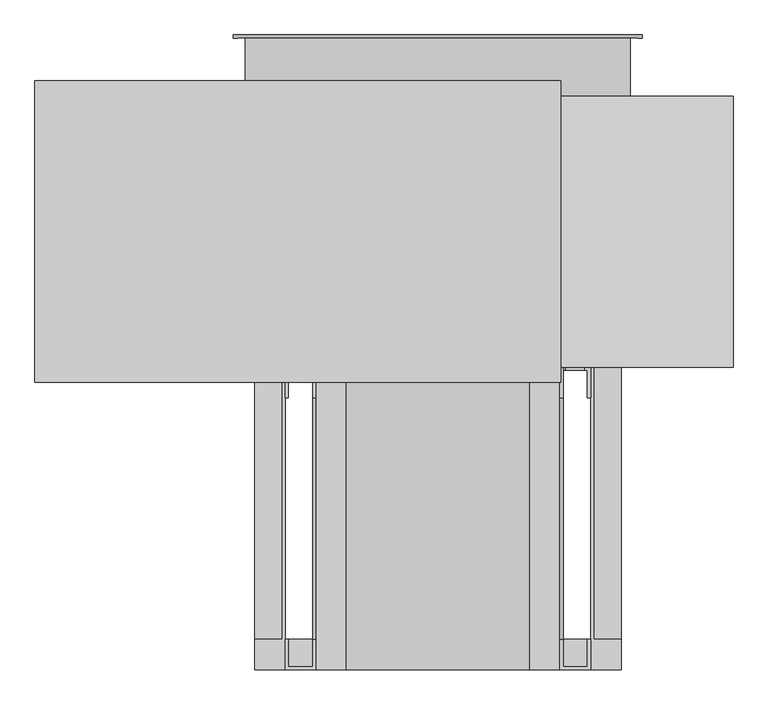
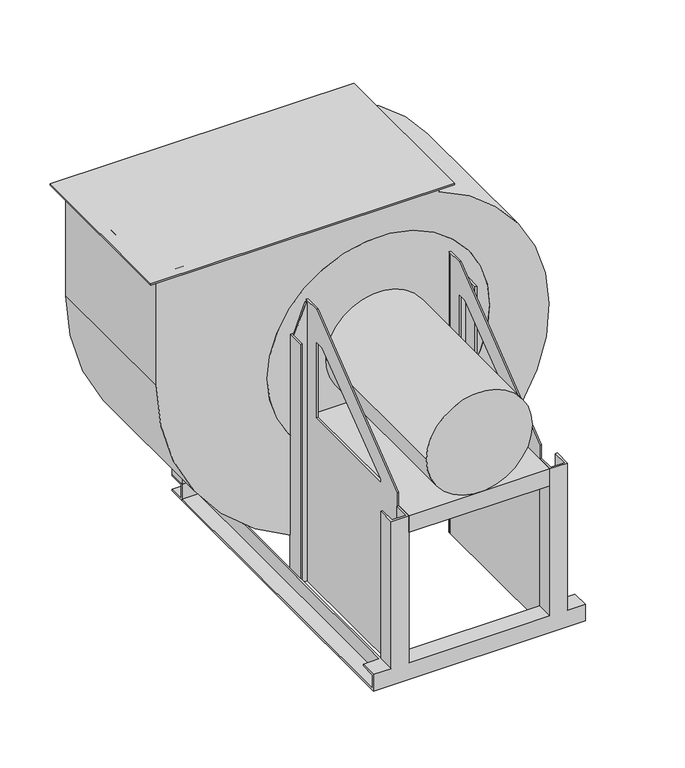
"""IFC4 building model written with IfcOpenShell, lengths in millimetres: proxy geometry, ВЕЗА_Вентилятор ВРАН : ВРАН9-063-ЛО."""

from ifc_helpers import new_model, si_unit, point, frame, frame_2d, origin, place, context, project, spatial, polyline, circle_curve, trimmed, segment, composite_curve, outline, extrude, faceted_brep, source, transform, mapped, element, save


def mechanical_equipment_c4a9a316(model_context):
    return source(origin(), model_context, "Body", "SolidModel", [
        extrude(outline(polyline([(201.5, -247.0), (-659.5, -247.0), (-659.5, 247.0), (201.5, 247.0), (201.5, -247.0)])), frame((0.0, 0.0, 1055.0), z_axis=(0.0, 0.0, 1.0), x_axis=(1.0, 0.0, 0.0)), (0.0, 0.0, 1.0), 5.0),
        extrude(outline(composite_curve([segment(trimmed(circle_curve(frame_2d((730.0, 5.524027)), 635.024027), [point((730.0, -629.5))], [point((95.0, 0.0))], False, "CARTESIAN"), True, "CONTINUOUS"), segment(trimmed(circle_curve(frame_2d((578.1699763, 0.3189338)), 483.1700816), [point((95.0, 0.0))], [point((1030.0, 171.5))], False, "CARTESIAN"), True, "CONTINUOUS"), segment(polyline([(1030.0, 171.5), (1060.0, 171.5), (1060.0, -629.5), (730.0, -629.5)]), True, "CONTINUOUS")], self_intersect=False), holes=[composite_curve([segment(trimmed(circle_curve(frame_2d((640.0, 0.0)), 315.0), [point((640.0, -315.0))], [point((640.0, 315.0))], True, "CARTESIAN"), True, "CONTINUOUS"), segment(trimmed(circle_curve(frame_2d((640.0, 0.0)), 315.0), [point((640.0, 315.0))], [point((640.0, -315.0))], True, "CARTESIAN"), True, "CONTINUOUS")], self_intersect=False)]), frame((0.0, -222.0, 0.0), z_axis=(0.0, 1.0, 0.0), x_axis=(0.0, 0.0, 1.0)), (0.0, 0.0, 1.0), 444.0),
        faceted_brep([(-300.0, -712.0, 5.0), (-300.0, 222.0, 5.0), (-300.0, 222.0, 0.0), (-300.0, -717.0, 0.0), (-300.0, -717.0, 50.0), (-300.0, -667.0, 50.0), (-300.0, -667.0, 45.0), (-300.0, -712.0, 45.0), (300.0, -717.0, 50.0), (300.0, -717.0, 0.0), (300.0, 222.0, 0.0), (300.0, 222.0, 5.0), (300.0, -712.0, 5.0), (300.0, -712.0, 45.0), (300.0, -667.0, 45.0), (300.0, -667.0, 50.0), (-250.0, 222.0, 0.0), (-250.0, -667.0, 0.0), (250.0, -667.0, 0.0), (250.0, 222.0, 0.0), (-255.0, -667.0, 50.0), (-255.0, -667.0, 45.0), (255.0, -667.0, 45.0), (255.0, -667.0, 50.0), (-200.0, -667.0, 490.0), (-200.0, -667.0, 50.0), (200.0, -667.0, 50.0), (200.0, -667.0, 490.0), (205.0, -667.0, 490.0), (205.0, -667.0, 50.0), (245.0, -667.0, 50.0), (245.0, -667.0, 490.0), (250.0, -667.0, 490.0), (250.0, -667.0, 50.0), (-250.0, -667.0, 50.0), (-250.0, -667.0, 490.0), (-245.0, -667.0, 490.0), (-245.0, -667.0, 50.0), (-205.0, -667.0, 50.0), (-205.0, -667.0, 490.0), (205.0, -667.0, 5.0), (245.0, -667.0, 5.0), (245.0, -667.0, 45.0), (205.0, -667.0, 45.0), (-245.0, -667.0, 5.0), (-205.0, -667.0, 5.0), (-205.0, -667.0, 45.0), (-245.0, -667.0, 45.0), (-200.0, -667.0, 5.0), (200.0, -667.0, 5.0), (200.0, -667.0, 45.0), (-200.0, -667.0, 45.0), (-255.0, -712.0, 5.0), (-255.0, 222.0, 5.0), (255.0, 222.0, 5.0), (255.0, -712.0, 5.0), (205.0, -712.0, 5.0), (245.0, -712.0, 5.0), (-245.0, -712.0, 5.0), (-205.0, -712.0, 5.0), (-200.0, -712.0, 5.0), (200.0, -712.0, 5.0), (255.0, -712.0, 45.0), (-255.0, -712.0, 45.0), (205.0, -712.0, 45.0), (245.0, -712.0, 45.0), (-245.0, -712.0, 45.0), (-205.0, -712.0, 45.0), (-200.0, -712.0, 45.0), (200.0, -712.0, 45.0), (255.0, 222.0, 50.0), (250.0, 222.0, 50.0), (250.0, -717.0, 50.0), (-250.0, -717.0, 50.0), (-250.0, 222.0, 50.0), (-255.0, 222.0, 50.0), (205.0, -712.0, 50.0), (245.0, -712.0, 50.0), (-245.0, -712.0, 50.0), (-205.0, -712.0, 50.0), (-200.0, -717.0, 50.0), (200.0, -717.0, 50.0), (250.0, -717.0, 490.0), (200.0, -717.0, 490.0), (-200.0, -717.0, 490.0), (-250.0, -717.0, 490.0), (245.0, -712.0, 490.0), (205.0, -712.0, 490.0), (-205.0, -712.0, 490.0), (-245.0, -712.0, 490.0)], [[[0, 1, 2, 3, 4, 5, 6, 7]], [[8, 9, 10, 11, 12, 13, 14, 15]], [[10, 9, 3, 2, 16, 17, 18, 19]], [[5, 20, 21, 6]], [[14, 22, 23, 15]], [[24, 25, 26, 27, 28, 29, 30, 31, 32, 33, 18, 17, 34, 35, 36, 37, 38, 39], [40, 41, 42, 43], [44, 45, 46, 47], [48, 49, 50, 51]], [[1, 0, 52, 53]], [[54, 55, 12, 11]], [[40, 56, 57, 41]], [[44, 58, 59, 45]], [[48, 60, 61, 49]], [[12, 55, 62, 13]], [[7, 63, 52, 0]], [[56, 64, 65, 57]], [[58, 66, 67, 59]], [[60, 68, 69, 61]], [[6, 21, 63, 7]], [[13, 62, 22, 14]], [[64, 43, 42, 65]], [[66, 47, 46, 67]], [[68, 51, 50, 69]], [[15, 23, 70, 71, 33, 72, 8]], [[4, 73, 34, 74, 75, 20, 5]], [[29, 76, 77, 30]], [[37, 78, 79, 38]], [[25, 80, 81, 26]], [[8, 72, 82, 83, 81, 80, 84, 85, 73, 4, 3, 9]], [[70, 54, 11, 10, 19, 71]], [[70, 23, 22, 62, 55, 54]], [[19, 18, 33, 71]], [[75, 74, 16, 2, 1, 53]], [[53, 52, 63, 21, 20, 75]], [[74, 34, 17, 16]], [[83, 82, 32, 31, 86, 87, 28, 27]], [[84, 24, 39, 88, 89, 36, 35, 85]], [[86, 77, 76, 87]], [[31, 30, 77, 86]], [[41, 57, 65, 42]], [[82, 72, 33, 32]], [[27, 26, 81, 83]], [[49, 61, 69, 50]], [[43, 64, 56, 40]], [[87, 76, 29, 28]], [[35, 34, 73, 85]], [[47, 66, 58, 44]], [[89, 78, 37, 36]], [[88, 79, 78, 89]], [[39, 38, 79, 88]], [[45, 59, 67, 46]], [[51, 68, 60, 48]], [[84, 80, 25, 24]]]),
        extrude(outline(polyline([(-667.0, 0.0), (-667.0, 530.0420316), (-272.0420316, 840.0), (-222.0, 840.0), (-222.0, 0.0), (-667.0, 0.0)]), holes=[polyline([(-272.0, 515.0), (-272.0, 740.0), (-296.9504813, 740.0), (-587.0, 521.5949723), (-587.0, 515.0), (-272.0, 515.0)])]), frame((-205.0, 0.0, 0.0), z_axis=(1.0, 0.0, 0.0), x_axis=(0.0, 1.0, 0.0)), (0.0, 0.0, 1.0), 5.0),
        faceted_brep([(250.0, 222.0, 50.0), (250.0, 227.0, 50.0), (295.0, 227.0, 50.0), (295.0, 272.0, 50.0), (300.0, 272.0, 50.0), (300.0, 222.0, 50.0), (300.0, 222.0, 485.0), (289.966699, 222.0, 485.0), (258.2904546, 222.0, 390.0), (250.0, 222.0, 390.0), (300.0, 272.0, 485.0), (295.0, 272.0, 485.0), (295.0, 227.0, 485.0), (250.0, 227.0, 390.0), (258.2904546, 227.0, 390.0), (289.966699, 227.0, 485.0)], [[[0, 1, 2, 3, 4, 5]], [[5, 6, 7, 8, 9, 0]], [[4, 10, 6, 5]], [[3, 11, 10, 4]], [[2, 12, 11, 3]], [[1, 13, 14, 15, 12, 2]], [[0, 9, 13, 1]], [[14, 13, 9, 8]], [[8, 7, 15, 14]], [[7, 6, 10, 11, 12, 15]]]),
        faceted_brep([(-250.0, 222.0, 50.0), (-300.0, 222.0, 50.0), (-300.0, 272.0, 50.0), (-295.0, 272.0, 50.0), (-295.0, 227.0, 50.0), (-250.0, 227.0, 50.0), (-250.0, 227.0, 390.0), (-250.0, 222.0, 390.0), (-295.0, 227.0, 485.0), (-289.966699, 227.0, 485.0), (-258.2904546, 227.0, 390.0), (-295.0, 272.0, 485.0), (-300.0, 272.0, 485.0), (-300.0, 222.0, 485.0), (-258.2904546, 222.0, 390.0), (-289.966699, 222.0, 485.0)], [[[0, 1, 2, 3, 4, 5]], [[5, 6, 7, 0]], [[4, 8, 9, 10, 6, 5]], [[3, 11, 8, 4]], [[2, 12, 11, 3]], [[1, 13, 12, 2]], [[0, 7, 14, 15, 13, 1]], [[9, 8, 11, 12, 13, 15]], [[15, 14, 10, 9]], [[14, 7, 6, 10]]]),
        extrude(outline(polyline([(-667.0, 0.0), (-667.0, 530.0420316), (-272.0420316, 840.0), (-222.0, 840.0), (-222.0, 0.0), (-667.0, 0.0)]), holes=[polyline([(-272.0, 515.0), (-272.0, 740.0), (-296.9504813, 740.0), (-587.0, 521.5949723), (-587.0, 515.0), (-272.0, 515.0)])]), frame((200.0, 0.0, 0.0), z_axis=(1.0, 0.0, 0.0), x_axis=(0.0, 1.0, 0.0)), (0.0, 0.0, 1.0), 5.0),
        faceted_brep([(200.0, -222.0, 0.0), (250.0, -222.0, 0.0), (250.0, -272.0, 0.0), (245.0, -272.0, 0.0), (245.0, -227.0, 0.0), (200.0, -227.0, 0.0), (200.0, -222.0, 833.6095143), (208.75409, -222.0, 833.6095143), (240.0, -222.0, 750.0), (250.0, -222.0, 750.0), (250.0, -272.0, 750.0), (245.0, -272.0, 750.0), (245.0, -227.0, 750.0), (240.0, -227.0, 750.0), (208.75409, -227.0, 833.6095143), (200.0, -227.0, 833.6095143)], [[[0, 1, 2, 3, 4, 5]], [[0, 6, 7, 8, 9, 1]], [[1, 9, 10, 2]], [[2, 10, 11, 3]], [[3, 11, 12, 4]], [[4, 12, 13, 14, 15, 5]], [[5, 15, 6, 0]], [[7, 6, 15, 14]], [[14, 13, 8, 7]], [[13, 12, 11, 10, 9, 8]]]),
        faceted_brep([(-200.0, -222.0, 0.0), (-200.0, -227.0, 0.0), (-245.0, -227.0, 0.0), (-245.0, -272.0, 0.0), (-250.0, -272.0, 0.0), (-250.0, -222.0, 0.0), (-200.0, -222.0, 833.6095143), (-200.0, -227.0, 833.6095143), (-208.75409, -227.0, 833.6095143), (-240.0, -227.0, 750.0), (-245.0, -227.0, 750.0), (-245.0, -272.0, 750.0), (-250.0, -272.0, 750.0), (-250.0, -222.0, 750.0), (-240.0, -222.0, 750.0), (-208.75409, -222.0, 833.6095143)], [[[0, 1, 2, 3, 4, 5]], [[0, 6, 7, 1]], [[1, 7, 8, 9, 10, 2]], [[2, 10, 11, 3]], [[3, 11, 12, 4]], [[4, 12, 13, 5]], [[5, 13, 14, 15, 6, 0]], [[14, 13, 12, 11, 10, 9]], [[9, 8, 15, 14]], [[8, 7, 6, 15]]]),
        extrude(outline(polyline([(222.0, 50.0), (272.0, 50.0), (272.0, 45.0), (227.0, 45.0), (227.0, 5.0), (272.0, 5.0), (272.0, 0.0), (222.0, 0.0), (222.0, 50.0)])), frame((-300.0, 0.0, 0.0), z_axis=(1.0, 0.0, 0.0), x_axis=(0.0, 1.0, 0.0)), (0.0, 0.0, 1.0), 600.0),
        extrude(outline(composite_curve([segment(trimmed(circle_curve(frame_2d((640.0, 0.0)), 315.0), [point((640.0, -315.0))], [point((640.0, 315.0))], False, "CARTESIAN"), True, "CONTINUOUS"), segment(trimmed(circle_curve(frame_2d((640.0, 0.0)), 315.0), [point((640.0, 315.0))], [point((640.0, -315.0))], False, "CARTESIAN"), True, "CONTINUOUS")], self_intersect=False)), frame((0.0, -222.0, 0.0), z_axis=(0.0, 1.0, 0.0), x_axis=(0.0, 0.0, 1.0)), (0.0, 0.0, 1.0), 5.0),
        extrude(outline(composite_curve([segment(trimmed(circle_curve(frame_2d((640.0, 0.0)), 335.0), [point((640.0, -335.0))], [point((640.0, 335.0))], False, "CARTESIAN"), True, "CONTINUOUS"), segment(trimmed(circle_curve(frame_2d((640.0, 0.0)), 335.0), [point((640.0, 335.0))], [point((640.0, -335.0))], False, "CARTESIAN"), True, "CONTINUOUS")], self_intersect=False), holes=[composite_curve([segment(trimmed(circle_curve(frame_2d((640.0, 0.0)), 305.0), [point((640.0, -305.0))], [point((640.0, 305.0))], True, "CARTESIAN"), True, "CONTINUOUS"), segment(trimmed(circle_curve(frame_2d((640.0, 0.0)), 305.0), [point((640.0, 305.0))], [point((640.0, -305.0))], True, "CARTESIAN"), True, "CONTINUOUS")], self_intersect=False)]), frame((0.0, 317.0, 0.0), z_axis=(0.0, 1.0, 0.0), x_axis=(0.0, 0.0, 1.0)), (0.0, 0.0, 1.0), 5.0),
        extrude(outline(polyline([(200.0, -717.0), (-200.0, -717.0), (-200.0, -222.0), (200.0, -222.0), (200.0, -717.0)])), frame((0.0, 0.0, 440.0), z_axis=(0.0, 0.0, 1.0), x_axis=(1.0, 0.0, 0.0)), (0.0, 0.0, 1.0), 50.0),
        extrude(outline(composite_curve([segment(trimmed(circle_curve(frame_2d((640.0, 0.0)), 150.0), [point((640.0, 150.0))], [point((640.0, -150.0))], False, "CARTESIAN"), True, "CONTINUOUS"), segment(trimmed(circle_curve(frame_2d((640.0, 0.0)), 150.0), [point((640.0, -150.0))], [point((640.0, 150.0))], False, "CARTESIAN"), True, "CONTINUOUS")], self_intersect=False)), frame((0.0, -717.0, 0.0), z_axis=(0.0, 1.0, 0.0), x_axis=(0.0, 0.0, 1.0)), (0.0, 0.0, 1.0), 495.0),
        extrude(outline(composite_curve([segment(trimmed(circle_curve(frame_2d((640.0, 0.0)), 315.0), [point((640.0, 315.0))], [point((640.0, -315.0))], False, "CARTESIAN"), True, "CONTINUOUS"), segment(trimmed(circle_curve(frame_2d((640.0, 0.0)), 315.0), [point((640.0, -315.0))], [point((640.0, 315.0))], False, "CARTESIAN"), True, "CONTINUOUS")], self_intersect=False), holes=[composite_curve([segment(trimmed(circle_curve(frame_2d((640.0, 0.0)), 305.0), [point((640.0, 305.0))], [point((640.0, -305.0))], True, "CARTESIAN"), True, "CONTINUOUS"), segment(trimmed(circle_curve(frame_2d((640.0, 0.0)), 305.0), [point((640.0, -305.0))], [point((640.0, 305.0))], True, "CARTESIAN"), True, "CONTINUOUS")], self_intersect=False)]), frame((0.0, 222.0, 0.0), z_axis=(0.0, 1.0, 0.0), x_axis=(0.0, 0.0, 1.0)), (0.0, 0.0, 1.0), 100.0),
    ])


if __name__ == "__main__":
    model = new_model("IFC4")
    model_context = context("Model", 3, world=origin())
    ifc_project = project(units=[si_unit("LENGTHUNIT", "METRE", prefix="MILLI")], contexts=[model_context])
    site = spatial("IfcSite", under=ifc_project)
    building = spatial("IfcBuilding", under=site)
    placement = place(None, origin())
    mechanical_equipment_shape = mechanical_equipment_c4a9a316(model_context)
    element("IfcBuildingElementProxy", 1, Name="ВЕЗА_Вентилятор ВРАН : ВРАН9-063-ЛО", ObjectType="ВЕЗА_Вентилятор ВРАН : ВРАН9-063-ЛО", at=placement, inside=building, context=model_context, shape_type="MappedRepresentation", body=[
        mapped(mechanical_equipment_shape, transform((0.0, 0.0, 0.0), x_axis=(1.0, 0.0, 0.0), y_axis=(0.0, 1.0, 0.0), z_axis=(0.0, 0.0, 1.0))),
    ])
    save(model, "model.ifc")

# Revit data of these elements
# Type "ВЕЗА_Вентилятор ВРАН : ВРАН9-063-ЛО"
#   УголВысота = "ВРАН_Угол_Высота"
#   ADSK_Этаж [instance default] = ""
#   ADSK_Примечание [instance default] = ""
#   ADSK_Позиция = "10"
#   ADSK_Обозначение = ""
#   ADSK_Наименование = "Вентилятор радиальный ВРАН6; типоразмер 063; режим работы Т80; исполнение коррозионностойкое; номинальная мощность Nном=4кВт, число -2007 полюсов 4; климатическое исполнение \r\nУХЛ2; конструктивное исполнение 1; положение корпуса ЛО; без ТШК"
#   О_Назначение [instance default] = ""
#   ADSK_Марка = "ВРАН6-063-Т80-К1 -00400/4-УХЛ2-1-ЛО-О ТУ 4861-104-40149153"
#   ADSK_Комплект [instance default] = ""
#   ADSK_Код изделия = "4044809"
#   ADSK_Зона [instance default] = ""
#   ADSK_Единица измерения = "компл."
#   И_НаименованиеФитинга = ""
#   И_НаименованиеСистемы [instance default] = ""
#   И_КодОборудования = "ВРАН9-063-ДУ"
#   ADSK_Завод-изготовитель = "ООО \"Веза\", Россия, Москва, ИНН 505001001, info@veza.ru"
#   Габариты = "vran_du"
#   ШиринаСтойкиОкна2 = 100 mm
#   ШиринаСтойкиОкна1 = 130 mm
#   ШиринаСтойкиДвигателя = 50 mm
#   Уголок = 50 mm
#   УголНаклона [instance default] = 0°
#   Угол [instance default] = 0°
#   Столик = -50 mm
#   Расход [instance default] = 0 m³/h
#   ADSK_Масса = 160
#   ADSK_Количество = 1
#   ADSK_Номинальная мощность [instance default] = 0 W
#   РадиусДвигателя = 150 mm
#   НомерВентилятора = 6.3 mm
#   ВысотаПлощадкиДвигателя [instance default] = 490 mm
#   ВерхОпор = 200 mm
#   R3 = 335 mm
#   R2 = 305 mm
#   Lmax = 989 mm
#   h [instance default] = 640 mm
#   R = 315 mm
#   L2 = 231 mm
#   H = 1066 mm
#   D = 630 mm
#   C = 550 mm
#   B_корпуса = 1140 mm
#   B = 802 mm
#   A = 444 mm
#   Швеллер = yes
#   Default Elevation = 0
#   Type Comments = ""
# Element 1 (IfcBuildingElementProxy, "ВЕЗА_Вентилятор ВРАН : ВРАН9-063-ЛО")
#   Расход = 4000 m³/h
#   ADSK_Номинальная мощность = 3000 W
